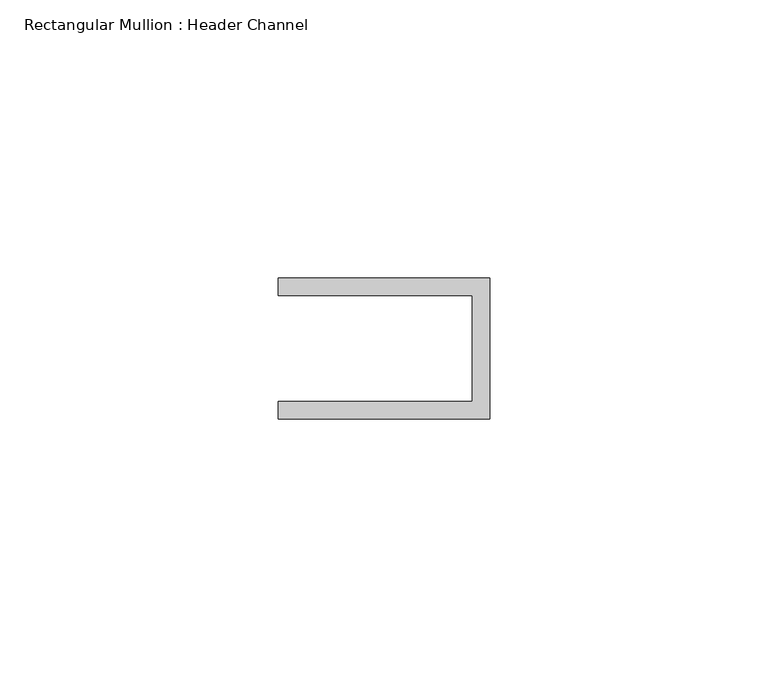
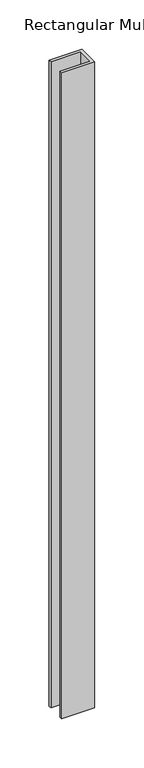
"""IFC4 building model written with IfcOpenShell, lengths in millimetres: member geometry, Rectangular Mullion : Header Channel."""

from ifc_helpers import new_model, si_unit, frame, origin, place, context, project, spatial, polyline, outline, extrude, source, transform, mapped, element, save


def rectangular_mullion_header_channel_ff144552(model_context):
    return source(origin(), model_context, "Body", "SweptSolid", [
        extrude(outline(polyline([(0.0, -12.7), (-38.1, -12.7), (-38.1, -9.525), (-3.175, -9.525), (-3.175, 9.525), (-38.1, 9.525), (-38.1, 12.7), (0.0, 12.7), (0.0, -12.7)])), frame((0.0, 0.0, -797.4591001), z_axis=(0.0, 0.0, 1.0), x_axis=(1.0, 0.0, 0.0)), (0.0, 0.0, 1.0), 797.4591001),
    ])


if __name__ == "__main__":
    model = new_model("IFC4")
    model_context = context("Model", 3, world=origin())
    ifc_project = project(units=[si_unit("LENGTHUNIT", "METRE", prefix="MILLI")], contexts=[model_context])
    site = spatial("IfcSite", under=ifc_project)
    building = spatial("IfcBuilding", under=site)
    placement = place(None, origin())
    rectangular_mullion_header_channel_shape = rectangular_mullion_header_channel_ff144552(model_context)
    element("IfcMember", 1, ObjectType="Rectangular Mullion : Header Channel", at=placement, inside=building, context=model_context, shape_type="MappedRepresentation", body=[
        mapped(rectangular_mullion_header_channel_shape, transform((0.0, 0.0, 0.0), x_axis=(1.0, 0.0, 0.0), y_axis=(0.0, 1.0, 0.0), z_axis=(0.0, 0.0, 1.0))),
    ])
    save(model, "model.ifc")

# Revit data of these elements
# Type "Rectangular Mullion : Header Channel"
#   built-in parameter 1007322 = 0.0833333 (stored number, unit not read)
#   built-in parameter 1007321 = -0.03125 (stored number, unit not read)
#   built-in parameter 1007320 = 0.0416667 (stored number, unit not read)
# Element 1 (IfcMember, "Rectangular Mullion : Header Channel")
#   Materials on its faces: "ALUM"
# Materials
#   "ALUM": class "Generic", colour RGB 157 157 157, transparency 0, Cost = 0
